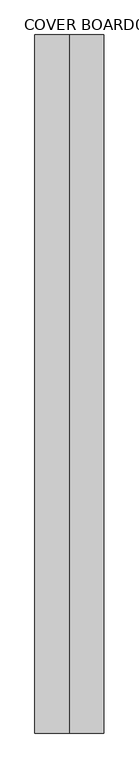
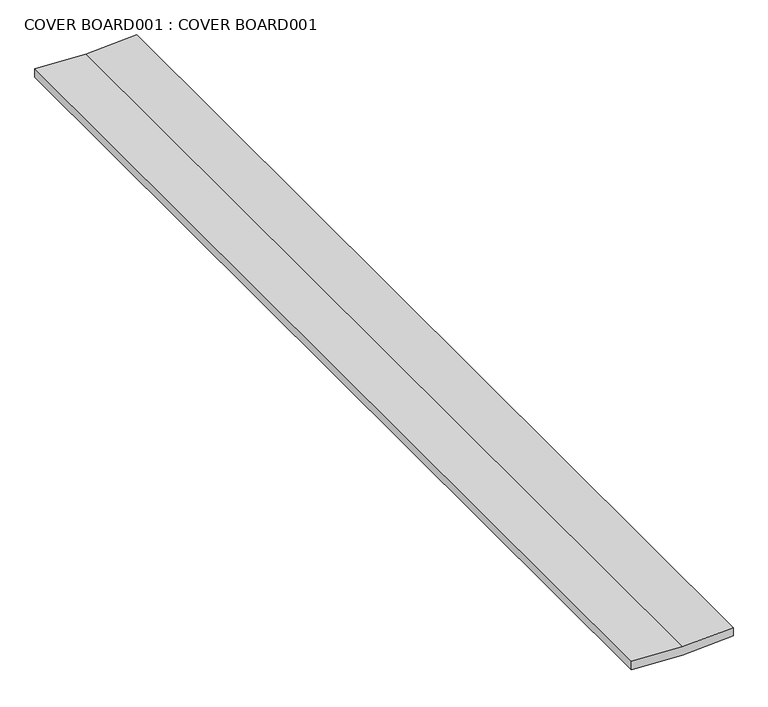
"""IFC4 building model written with IfcOpenShell, lengths in millimetres: proxy geometry, COVER BOARD001 : COVER BOARD001."""

from ifc_helpers import new_model, si_unit, frame, origin, place, context, project, spatial, polyline, outline, extrude, source, transform, mapped, element, save


def cover_board001_cover_board001_0c3f8cb2(model_context):
    return source(origin(), model_context, "Body", "SweptSolid", [
        extrude(outline(polyline([(40232.8984375, -4699.8063764), (40237.9000089, -4797.9038825), (40220.5682898, -4797.9038825), (40215.5667183, -4699.8063764), (40220.5682898, -4601.0538825), (40237.9000089, -4601.0538825), (40232.8984375, -4699.8063764)])), frame((0.0, -1052.6406573, 0.0), z_axis=(0.0, 1.0, 0.0), x_axis=(0.0, 0.0, 1.0)), (0.0, 0.0, 1.0), 2000.0),
    ])


if __name__ == "__main__":
    model = new_model("IFC4")
    model_context = context("Model", 3, world=origin())
    ifc_project = project(units=[si_unit("LENGTHUNIT", "METRE", prefix="MILLI")], contexts=[model_context])
    site = spatial("IfcSite", under=ifc_project)
    building = spatial("IfcBuilding", under=site)
    placement = place(None, origin())
    cover_board001_cover_board001_shape = cover_board001_cover_board001_0c3f8cb2(model_context)
    element("IfcBuildingElementProxy", 1, Name="COVER BOARD001 : COVER BOARD001", ObjectType="COVER BOARD001 : COVER BOARD001", at=placement, inside=building, context=model_context, shape_type="MappedRepresentation", body=[
        mapped(cover_board001_cover_board001_shape, transform((0.0, 0.0, 0.0), x_axis=(1.0, 0.0, 0.0), y_axis=(0.0, 1.0, 0.0), z_axis=(0.0, 0.0, 1.0))),
    ])
    save(model, "model.ifc")

# Revit data of these elements
# Type "COVER BOARD001 : COVER BOARD001"
#   NameOverride = "COVER BOARD001"
# Element 1 (IfcBuildingElementProxy, "COVER BOARD001 : COVER BOARD001")
#   Materials on its faces: "CDX PLYWOOD - SEE STRUCTURAL DWGS"
# Materials
#   "CDX PLYWOOD - SEE STRUCTURAL DWGS": class "Unassigned", colour RGB 177 130 114, transparency 0, Cost = 0
